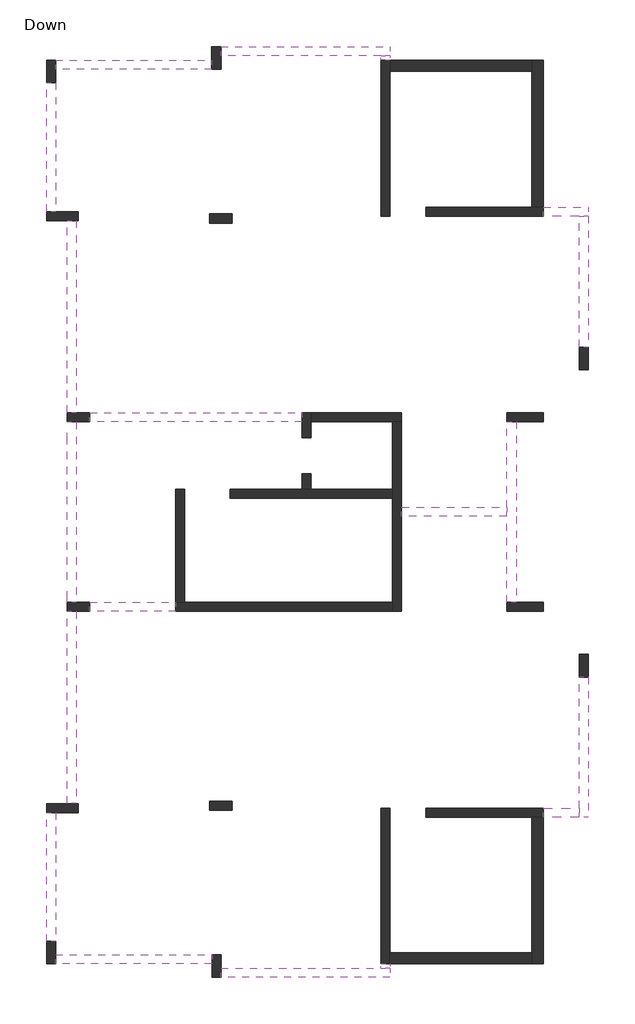
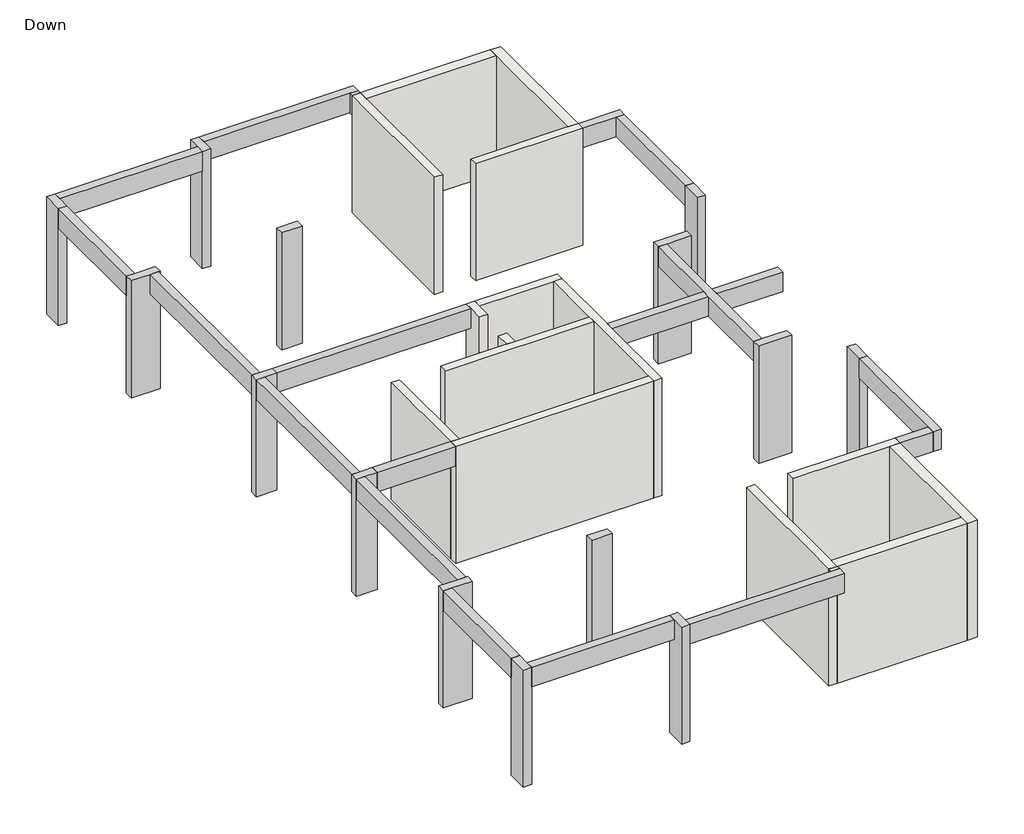
# One storey: 19 beams, 15 walls, 14 columns.
"""IFC4 building model written with IfcOpenShell, lengths in millimetres."""

from ifc_helpers import new_model, si_unit, origin, origin_with_axes, place, context, project, spatial, polyline, outline, extrude, faceted_brep, element, save

model = new_model("IFC4")

# Units and contexts
model_context = context("Model", 3, world=origin())
ifc_project = project(units=[si_unit("LENGTHUNIT", "METRE", prefix="MILLI")], contexts=[model_context])

# Site, building, storey
site = spatial("IfcSite", under=ifc_project)
building = spatial("IfcBuilding", under=site)
storey = spatial("IfcBuildingStorey", under=building, Name="Down", Elevation=0.0)

# Beams
placement = place(None, origin())
element("IfcBeam", 1, ObjectType="Concrete Rectengular Beam : 20/50", at=placement, inside=storey, context=model_context, shape_type="Brep", body=[
    faceted_brep([(-1347.6312201, 19838.1909584, 3000.0), (-1547.6312201, 19838.1909584, 3000.0), (-1547.6312201, 16987.4100295, 3000.0), (-1347.6312201, 16987.4100295, 3000.0), (-1547.6312201, 19838.1909584, 2500.0), (-1547.6312201, 16987.4100295, 2500.0), (-1347.6312201, 19838.1909584, 2500.0), (-1347.6312201, 16987.4100295, 2500.0), (-1347.6312201, 16987.4100295, 2800.0)], [[[0, 1, 2, 3]], [[1, 4, 5, 2]], [[4, 6, 7, 5]], [[6, 0, 3, 8, 7]], [[1, 0, 6, 4]], [[3, 2, 5, 7, 8]]]),
])
element("IfcBeam", 2, ObjectType="Concrete Rectengular Beam : 20/50", at=placement, inside=storey, context=model_context, shape_type="Brep", body=[
    faceted_brep([(-1086.1844466, 12537.0195651, 3000.0), (-886.1844466, 12537.0195651, 3000.0), (-886.1844466, 16787.4100295, 3000.0), (-1086.1844466, 16787.4100295, 3000.0), (-886.1844466, 12537.0195651, 2800.0), (-886.1844466, 12537.0195651, 2500.0), (-886.1844466, 16787.4100295, 2500.0), (-886.1844466, 16787.4100295, 2800.0), (-1086.1844466, 12537.0195651, 2500.0), (-1086.1844466, 16787.4100295, 2500.0), (-1086.1844466, 16787.4100295, 2800.0)], [[[0, 1, 2, 3]], [[2, 1, 4, 5, 6, 7]], [[5, 8, 9, 6]], [[3, 10, 9, 8, 0]], [[1, 0, 8, 5, 4]], [[3, 2, 7, 6, 9, 10]]]),
])
element("IfcBeam", 3, ObjectType="Concrete Rectengular Beam : 20/50", at=placement, inside=storey, context=model_context, shape_type="Brep", body=[
    faceted_brep([(-886.1844466, 12337.0195651, 3000.0), (-1086.1844466, 12337.0195651, 3000.0), (-1086.1844466, 11837.4100295, 3000.0), (-1086.1844466, 8836.9784636, 3000.0), (-1086.1844466, 8336.34139, 3000.0), (-886.1844466, 8336.34139, 3000.0), (-1086.1844466, 12337.0195651, 2500.0), (-1086.1844466, 8336.34139, 2500.0), (-886.1844466, 12337.0195651, 2500.0), (-886.1844466, 8336.34139, 2500.0), (-886.1844466, 12337.0195651, 2800.0), (-886.1844466, 8336.34139, 2800.0)], [[[0, 1, 2, 3, 4, 5]], [[1, 6, 7, 4, 3, 2]], [[6, 8, 9, 7]], [[8, 10, 0, 5, 11, 9]], [[1, 0, 10, 8, 6]], [[5, 4, 7, 9, 11]]]),
])
element("IfcBeam", 4, ObjectType="Concrete Rectengular Beam : 20/50", at=placement, inside=storey, context=model_context, shape_type="Brep", body=[
    faceted_brep([(-1086.1844466, 3886.9784636, 3000.0), (-886.1844466, 3886.9784636, 3000.0), (-886.1844466, 8136.34139, 3000.0), (-1086.1844466, 8136.34139, 3000.0), (-1086.1844466, 3886.9784636, 2500.0), (-1086.1844466, 3886.9784636, 2800.0), (-1086.1844466, 8136.34139, 2500.0), (-886.1844466, 3886.9784636, 2500.0), (-886.1844466, 8136.34139, 2500.0), (-886.1844466, 3886.9784636, 2800.0), (-886.1844466, 8136.34139, 2800.0)], [[[0, 1, 2, 3]], [[4, 5, 0, 3, 6]], [[7, 4, 6, 8]], [[2, 1, 9, 7, 8, 10]], [[3, 2, 10, 8, 6]], [[1, 0, 5, 4, 7, 9]]]),
])
element("IfcBeam", 5, ObjectType="Concrete Rectengular Beam : 20/50", at=placement, inside=storey, context=model_context, shape_type="Brep", body=[
    faceted_brep([(-1547.6312201, 836.1975347, 3000.0), (-1347.6312201, 836.1975347, 3000.0), (-1347.6312201, 3686.9784636, 3000.0), (-1547.6312201, 3686.9784636, 3000.0), (-1547.6312201, 3686.5951919, 3000.0), (-1347.6312201, 836.1975347, 2500.0), (-1347.6312201, 3686.9784636, 2500.0), (-1347.6312201, 3686.9784636, 2800.0), (-1547.6312201, 836.1975347, 2500.0), (-1547.6312201, 3686.9784636, 2500.0), (-1547.6312201, 3686.9784636, 2800.0)], [[[0, 1, 2, 3, 4]], [[1, 5, 6, 7, 2]], [[5, 8, 9, 6]], [[8, 0, 4, 3, 10, 9]], [[1, 0, 8, 5]], [[3, 2, 7, 6, 9, 10]]]),
])
element("IfcBeam", 6, ObjectType="Concrete Rectengular Beam : 20/50", at=placement, inside=storey, context=model_context, shape_type="Brep", body=[
    faceted_brep([(-1347.6312201, 537.7388417, 3000.0), (-1347.6312201, 337.7388417, 3000.0), (2114.3087716, 337.7388417, 3000.0), (2114.3087716, 537.7388417, 3000.0), (2114.3087716, 537.7388417, 2800.0), (2114.3087716, 537.7388417, 2500.0), (-1347.6312201, 537.7388417, 2500.0), (-1347.6312201, 537.7388417, 2800.0), (-1347.6312201, 337.7388417, 2500.0), (2114.3087716, 337.7388417, 2500.0)], [[[0, 1, 2, 3]], [[0, 3, 4, 5, 6, 7]], [[8, 6, 5, 9]], [[1, 8, 9, 2]], [[1, 0, 7, 6, 8]], [[3, 2, 9, 5, 4]]]),
])
element("IfcBeam", 7, ObjectType="Concrete Rectengular Beam : 20/50", at=placement, inside=storey, context=model_context, shape_type="Brep", body=[
    faceted_brep([(6055.3348071, 37.7388417, 3000.0), (6055.3348071, 237.7388417, 3000.0), (5855.3348071, 237.7388417, 3000.0), (2314.3087716, 237.7388417, 3000.0), (2314.3087716, 37.7388417, 3000.0), (6055.3348071, 37.7388417, 2500.0), (2314.3087716, 37.7388417, 2500.0), (6055.3348071, 237.7388417, 2500.0), (2314.3087716, 237.7388417, 2500.0), (5855.3348071, 237.7388417, 2500.0)], [[[0, 1, 2, 3, 4]], [[5, 0, 4, 6]], [[7, 5, 6, 8, 9]], [[1, 7, 9, 8, 3, 2]], [[4, 3, 8, 6]], [[1, 0, 5, 7]]]),
])
element("IfcBeam", 8, ObjectType="Concrete Rectengular Beam : 20/50", at=placement, inside=storey, context=model_context, shape_type="Brep", body=[
    faceted_brep([(2113.2812336, 20138.1909584, 3000.0), (2113.2812336, 20338.1909584, 3000.0), (-1347.6312201, 20338.1909584, 3000.0), (-1347.6312201, 20138.1909584, 3000.0), (2113.2812336, 20138.1909584, 2500.0), (2113.2812336, 20138.1909584, 2800.0), (-1347.6312201, 20138.1909584, 2800.0), (-1347.6312201, 20138.1909584, 2500.0), (2113.2812336, 20338.1909584, 2500.0), (-1347.6312201, 20338.1909584, 2500.0)], [[[0, 1, 2, 3]], [[4, 5, 0, 3, 6, 7]], [[8, 4, 7, 9]], [[1, 8, 9, 2]], [[1, 0, 5, 4, 8]], [[3, 2, 9, 7, 6]]]),
])
element("IfcBeam", 9, ObjectType="Concrete Rectengular Beam : 20/50", at=placement, inside=storey, context=model_context, shape_type="Brep", body=[
    faceted_brep([(6055.3348071, 20438.1909584, 3000.0), (6055.3348071, 20638.1909584, 3000.0), (2313.2812336, 20638.1909584, 3000.0), (2313.2812336, 20438.1909584, 3000.0), (5855.3348071, 20438.1909584, 3000.0), (6055.3348071, 20438.1909584, 2500.0), (2313.2812336, 20438.1909584, 2800.0), (2313.2812336, 20438.1909584, 2500.0), (5855.3348071, 20438.1909584, 2500.0), (6055.3348071, 20638.1909584, 2500.0), (2313.2812336, 20638.1909584, 2500.0)], [[[0, 1, 2, 3, 4]], [[5, 0, 4, 3, 6, 7, 8]], [[9, 5, 8, 7, 10]], [[1, 9, 10, 2]], [[3, 2, 10, 7, 6]], [[1, 0, 5, 9]]]),
])
element("IfcBeam", 10, ObjectType="Concrete Rectengular Beam : 20/50", at=placement, inside=storey, context=model_context, shape_type="Brep", body=[
    faceted_brep([(6055.3348071, 20438.1909584, 3000.0), (5855.3348071, 20438.1909584, 3000.0), (5855.3348071, 20337.1634204, 3000.0), (6055.3348071, 20337.1634204, 3000.0), (6055.3348071, 20438.1909584, 2500.0), (6055.3348071, 20337.1634204, 2500.0), (5855.3348071, 20438.1909584, 2500.0), (5855.3348071, 20337.1634204, 2500.0), (5855.3348071, 20438.1909584, 2800.0), (5855.3348071, 20337.1634204, 2800.0)], [[[0, 1, 2, 3]], [[4, 0, 3, 5]], [[6, 4, 5, 7]], [[2, 1, 8, 6, 7, 9]], [[1, 0, 4, 6, 8]], [[3, 2, 9, 7, 5]]]),
])
element("IfcBeam", 11, ObjectType="Concrete Rectengular Beam : 20/50", at=placement, inside=storey, context=model_context, shape_type="Brep", body=[
    faceted_brep([(5855.3348071, 237.7388417, 3000.0), (6055.3348071, 237.7388417, 3000.0), (6055.3348071, 336.1975347, 3000.0), (5855.3348071, 336.1975347, 3000.0), (5855.3348071, 336.1975347, 2800.0), (5855.3348071, 336.1975347, 2500.0), (5855.3348071, 237.7388417, 2500.0), (5855.3348071, 237.7388417, 2800.0), (6055.3348071, 237.7388417, 2500.0), (6055.3348071, 336.1975347, 2500.0)], [[[0, 1, 2, 3]], [[0, 3, 4, 5, 6, 7]], [[8, 6, 5, 9]], [[1, 8, 9, 2]], [[1, 0, 7, 6, 8]], [[3, 2, 9, 5, 4]]]),
])
element("IfcBeam", 12, ObjectType="Concrete Rectengular Beam : 20/50", at=placement, inside=storey, context=model_context, shape_type="Brep", body=[
    faceted_brep([(9453.0058534, 17086.8962605, 3000.0), (9453.0058534, 16886.8962605, 3000.0), (10255.2560168, 16886.8962605, 3000.0), (10455.2560168, 16886.8962605, 3000.0), (10455.2560168, 17086.8962605, 3000.0), (9453.0058534, 17086.8962605, 2500.0), (10455.2560168, 17086.8962605, 2500.0), (9453.0058534, 16886.8962605, 2500.0), (10455.2560168, 16886.8962605, 2500.0), (10255.2560168, 16886.8962605, 2500.0), (9453.0058534, 16886.8962605, 2800.0)], [[[0, 1, 2, 3, 4]], [[5, 0, 4, 6]], [[7, 5, 6, 8, 9]], [[8, 3, 2, 1, 10, 7, 9]], [[1, 0, 5, 7, 10]], [[4, 3, 8, 6]]]),
])
element("IfcBeam", 13, ObjectType="Concrete Rectengular Beam : 20/50", at=placement, inside=storey, context=model_context, shape_type="Brep", body=[
    faceted_brep([(-586.1844466, 8336.34139, 3000.0), (-586.1844466, 8136.34139, 3000.0), (1314.1854671, 8136.34139, 3000.0), (1314.1854671, 8336.34139, 3000.0), (-586.1844466, 8136.34139, 2800.0), (-586.1844466, 8136.34139, 2500.0), (1314.1854671, 8136.34139, 2500.0), (1314.1854671, 8136.34139, 2800.0), (-586.1844466, 8336.34139, 2500.0), (1314.1854671, 8336.34139, 2500.0), (1314.1854671, 8336.34139, 2800.0)], [[[0, 1, 2, 3]], [[2, 1, 4, 5, 6, 7]], [[5, 8, 9, 6]], [[8, 0, 3, 10, 9]], [[1, 0, 8, 5, 4]], [[3, 2, 7, 6, 9, 10]]]),
])
element("IfcBeam", 14, ObjectType="Concrete Rectengular Beam : 20/50", at=placement, inside=storey, context=model_context, shape_type="Brep", body=[
    faceted_brep([(-586.1844466, 12537.0195651, 3000.0), (-586.1844466, 12337.0195651, 3000.0), (4114.617033, 12337.0195651, 3000.0), (4114.617033, 12537.0195651, 3000.0), (-586.1844466, 12337.0195651, 2500.0), (4114.617033, 12337.0195651, 2500.0), (4114.617033, 12337.0195651, 2800.0), (-586.1844466, 12537.0195651, 2500.0), (4114.617033, 12537.0195651, 2500.0), (4114.617033, 12537.0195651, 2800.0), (-586.1844466, 12537.0195651, 2800.0)], [[[0, 1, 2, 3]], [[1, 4, 5, 6, 2]], [[4, 7, 8, 5]], [[0, 3, 9, 8, 7, 10]], [[1, 0, 10, 7, 4]], [[3, 2, 6, 5, 8, 9]]]),
])
element("IfcBeam", 15, ObjectType="Concrete Rectengular Beam : 20/50", at=placement, inside=storey, context=model_context, shape_type="Brep", body=[
    faceted_brep([(10255.2458863, 3586.4646946, 3000.0), (10455.2458863, 3586.4646946, 3000.0), (10455.2458863, 6686.3824915, 3000.0), (10255.2458863, 6686.3824915, 3000.0), (10255.2458863, 3786.4646946, 3000.0), (10255.2458863, 3586.4646946, 2500.0), (10255.2458863, 6686.3824915, 2500.0), (10255.2458863, 3786.4646946, 2500.0), (10455.2458863, 3586.4646946, 2500.0), (10455.2458863, 6686.3824915, 2500.0)], [[[0, 1, 2, 3, 4]], [[5, 0, 4, 3, 6, 7]], [[8, 5, 7, 6, 9]], [[1, 8, 9, 2]], [[3, 2, 9, 6]], [[1, 0, 5, 8]]]),
])
element("IfcBeam", 16, ObjectType="Concrete Rectengular Beam : 20/50", at=placement, inside=storey, context=model_context, shape_type="Brep", body=[
    faceted_brep([(10255.2458863, 3586.4646946, 3000.0), (10255.2458863, 3786.4646946, 3000.0), (9453.0058534, 3786.4646946, 3000.0), (9453.0058534, 3586.4646946, 3000.0), (10255.2458863, 3786.4646946, 2800.0), (10255.2458863, 3786.4646946, 2500.0), (9453.0058534, 3786.4646946, 2500.0), (9453.0058534, 3786.4646946, 2800.0), (10255.2458863, 3586.4646946, 2500.0), (9453.0058534, 3586.4646946, 2500.0)], [[[0, 1, 2, 3]], [[2, 1, 4, 5, 6, 7]], [[5, 8, 9, 6]], [[8, 0, 3, 9]], [[1, 0, 8, 5, 4]], [[3, 2, 7, 6, 9]]]),
])
element("IfcBeam", 17, ObjectType="Concrete Rectengular Beam : 20/50", at=placement, inside=storey, context=model_context, shape_type="Brep", body=[
    faceted_brep([(8852.8825489, 12337.0195651, 3000.0), (8652.8825489, 12337.0195651, 3000.0), (8652.8825489, 10438.2526107, 3000.0), (8652.8825489, 10238.2526107, 3000.0), (8652.8825489, 8336.34139, 3000.0), (8852.561957, 8336.34139, 3000.0), (8852.561957, 10238.2526107, 3000.0), (8852.8825489, 10238.2526107, 3000.0), (8852.8825489, 10438.2526107, 3000.0), (8852.8825489, 8336.34139, 2500.0), (8852.8825489, 10238.2526107, 2500.0), (8852.8825489, 10438.2526107, 2500.0), (8852.8825489, 12337.0195651, 2500.0), (8852.8825489, 12337.0195651, 2800.0), (8852.8825489, 10238.2526107, 2800.0), (8852.8825489, 8336.34139, 2800.0), (8652.8825489, 8336.34139, 2500.0), (8652.8825489, 10238.2526107, 2500.0), (8652.8825489, 10438.2526107, 2500.0), (8652.8825489, 12337.0195651, 2500.0), (8652.8825489, 8336.34139, 2800.0), (8652.8825489, 12337.0195651, 2800.0), (8852.561957, 8336.34139, 2800.0), (8852.561957, 10238.2526107, 2800.0)], [[[0, 1, 2, 3, 4, 5, 6, 7, 8]], [[9, 10, 11, 12, 13, 0, 8, 7, 14, 15]], [[9, 16, 17, 18, 19, 12, 11, 10]], [[19, 18, 17, 16, 20, 4, 3, 2, 1, 21]], [[16, 9, 15, 22, 5, 4, 20]], [[1, 0, 13, 12, 19, 21]], [[23, 22, 15, 14]], [[22, 23, 6, 5]], [[6, 23, 14, 7]]]),
])
element("IfcBeam", 18, ObjectType="Concrete Rectengular Beam : 20/50", at=placement, inside=storey, context=model_context, shape_type="Brep", body=[
    faceted_brep([(10453.8977564, 10238.2526107, 3000.0), (10453.8977564, 10238.2526107, 2800.0), (10453.8977564, 10238.2526107, 2500.0), (10453.8977564, 10438.2526107, 2500.0), (10453.8977564, 10438.2526107, 2800.0), (10453.8977564, 10438.2526107, 3000.0), (8852.8825489, 10238.2526107, 3000.0), (8852.8825489, 10438.2526107, 3000.0), (8852.8825489, 10438.2526107, 2800.0), (8852.8825489, 10438.2526107, 2500.0), (8852.8825489, 10238.2526107, 2500.0), (8852.8825489, 10238.2526107, 2800.0)], [[[0, 1, 2, 3, 4, 5]], [[6, 7, 8, 9, 10, 11]], [[0, 5, 7, 6]], [[5, 4, 3, 9, 8, 7]], [[3, 2, 10, 9]], [[2, 1, 0, 6, 11, 10]]]),
    faceted_brep([(6313.8977564, 10438.2526107, 3000.0), (6313.8977564, 10238.2526107, 3000.0), (8652.8825489, 10238.2526107, 3000.0), (8652.8825489, 10438.2526107, 3000.0), (6313.8977564, 10438.2526107, 2500.0), (6313.8977564, 10438.2526107, 2800.0), (8652.8825489, 10438.2526107, 2800.0), (8652.8825489, 10438.2526107, 2500.0), (6313.8977564, 10238.2526107, 2500.0), (8652.8825489, 10238.2526107, 2500.0)], [[[0, 1, 2, 3]], [[4, 5, 0, 3, 6, 7]], [[8, 4, 7, 9]], [[1, 8, 9, 2]], [[1, 0, 5, 4, 8]], [[3, 2, 9, 7, 6]]]),
])
element("IfcBeam", 19, ObjectType="Concrete Rectengular Beam : 20/50", at=placement, inside=storey, context=model_context, shape_type="Brep", body=[
    faceted_brep([(10255.2560168, 13985.039794, 3000.0), (10455.2560168, 13985.039794, 3000.0), (10455.2560168, 16886.8962605, 3000.0), (10255.2560168, 16886.8962605, 3000.0), (10455.2560168, 13985.039794, 2500.0), (10455.2560168, 16886.8962605, 2500.0), (10255.2560168, 13985.039794, 2500.0), (10255.2560168, 16886.8962605, 2500.0), (10255.2560168, 16886.8962605, 2800.0)], [[[0, 1, 2, 3]], [[1, 4, 5, 2]], [[4, 6, 7, 5]], [[6, 0, 3, 8, 7]], [[1, 0, 6, 4]], [[3, 2, 5, 7, 8]]]),
])

# Columns
element("IfcColumn", 20, ObjectType="Concrete Rectengular Column : 20/50", at=placement, inside=storey, context=model_context, shape_type="Brep", body=[
    faceted_brep([(-1347.6312201, 20338.1909584, 0.0), (-1347.6312201, 19838.1909584, 0.0), (-1547.6312201, 19838.1909584, 0.0), (-1547.6312201, 20338.1909584, 0.0), (-1347.6312201, 20338.1909584, 3000.0), (-1347.6312201, 20138.1909584, 3000.0), (-1347.6312201, 19838.1909584, 3000.0), (-1547.6312201, 19838.1909584, 3000.0), (-1547.6312201, 20338.1909584, 3000.0)], [[[0, 1, 2, 3]], [[4, 5, 6, 1, 0]], [[6, 7, 2, 1]], [[7, 8, 3, 2]], [[8, 4, 0, 3]], [[4, 8, 7, 6, 5]]]),
])
element("IfcColumn", 21, ObjectType="Concrete Rectengular Column : 20/50", at=placement, inside=storey, context=model_context, shape_type="Brep", body=[
    faceted_brep([(2313.2812336, 20638.1909584, 0.0), (2313.2812336, 20138.1909584, 0.0), (2113.2812336, 20138.1909584, 0.0), (2113.2812336, 20638.1909584, 0.0), (2313.2812336, 20638.1909584, 3000.0), (2313.2812336, 20438.1909584, 3000.0), (2313.2812336, 20138.1909584, 3000.0), (2313.2812336, 20138.1909584, 2800.0), (2113.2812336, 20138.1909584, 3000.0), (2113.2812336, 20638.1909584, 3000.0)], [[[0, 1, 2, 3]], [[4, 5, 6, 7, 1, 0]], [[6, 8, 2, 1, 7]], [[8, 9, 3, 2]], [[9, 4, 0, 3]], [[4, 9, 8, 6, 5]]]),
])
element("IfcColumn", 22, ObjectType="Concrete Rectengular Column : 20/50", at=placement, inside=storey, context=model_context, shape_type="Brep", body=[
    faceted_brep([(2063.507292, 16933.4642836, 0.0), (2563.507292, 16933.4642836, 0.0), (2563.507292, 16733.4642836, 0.0), (2063.507292, 16733.4642836, 0.0), (2063.507292, 16933.4642836, 3000.0), (2563.507292, 16933.4642836, 3000.0), (2563.507292, 16933.4642836, 2800.0), (2063.507292, 16933.4642836, 2800.0), (2563.507292, 16733.4642836, 3000.0), (2563.507292, 16733.4642836, 2800.0), (2063.507292, 16733.4642836, 3000.0), (2063.507292, 16733.4642836, 2800.0)], [[[0, 1, 2, 3]], [[4, 5, 6, 1, 0, 7]], [[5, 8, 9, 2, 1, 6]], [[8, 10, 11, 3, 2, 9]], [[10, 4, 7, 0, 3, 11]], [[4, 10, 8, 5]]]),
])
element("IfcColumn", 23, ObjectType="Concrete Rectengular Column : 20/50", at=placement, inside=storey, context=model_context, shape_type="Brep", body=[
    faceted_brep([(-1086.1844466, 12537.0195651, 0.0), (-586.1844466, 12537.0195651, 0.0), (-586.1844466, 12337.0195651, 0.0), (-1086.1844466, 12337.0195651, 0.0), (-1086.1844466, 12537.0195651, 3000.0), (-886.1844466, 12537.0195651, 3000.0), (-586.1844466, 12537.0195651, 3000.0), (-586.1844466, 12337.0195651, 3000.0), (-886.1844466, 12337.0195651, 3000.0), (-1086.1844466, 12337.0195651, 3000.0)], [[[0, 1, 2, 3]], [[4, 5, 6, 1, 0]], [[6, 7, 2, 1]], [[7, 8, 9, 3, 2]], [[9, 4, 0, 3]], [[4, 9, 8, 7, 6, 5]]]),
])
element("IfcColumn", 24, ObjectType="Concrete Rectengular Column : 20/50", at=placement, inside=storey, context=model_context, shape_type="Brep", body=[
    faceted_brep([(-1086.1844466, 8336.34139, 0.0), (-586.1844466, 8336.34139, 0.0), (-586.1844466, 8136.34139, 0.0), (-1086.1844466, 8136.34139, 0.0), (-1086.1844466, 8336.34139, 3000.0), (-886.1844466, 8336.34139, 3000.0), (-586.1844466, 8336.34139, 3000.0), (-586.1844466, 8136.34139, 3000.0), (-886.3077512, 8136.34139, 3000.0), (-1086.1844466, 8136.34139, 3000.0)], [[[0, 1, 2, 3]], [[4, 5, 6, 1, 0]], [[6, 7, 2, 1]], [[7, 8, 9, 3, 2]], [[9, 4, 0, 3]], [[4, 9, 8, 7, 6, 5]]]),
])
element("IfcColumn", 25, ObjectType="Concrete Rectengular Column : 20/50", at=placement, inside=storey, context=model_context, shape_type="Brep", body=[
    faceted_brep([(-1547.6312201, 336.1975347, 0.0), (-1547.6312201, 836.1975347, 0.0), (-1347.6312201, 836.1975347, 0.0), (-1347.6312201, 336.1975347, 0.0), (-1547.6312201, 336.1975347, 3000.0), (-1547.6312201, 836.1975347, 3000.0), (-1347.6312201, 836.1975347, 3000.0), (-1347.6312201, 537.7388417, 3000.0), (-1347.6312201, 336.1975347, 3000.0)], [[[0, 1, 2, 3]], [[4, 5, 1, 0]], [[5, 6, 2, 1]], [[6, 7, 8, 3, 2]], [[8, 4, 0, 3]], [[4, 8, 7, 6, 5]]]),
])
element("IfcColumn", 26, ObjectType="Concrete Rectengular Column : 20/50", at=placement, inside=storey, context=model_context, shape_type="Brep", body=[
    faceted_brep([(2566.6823845, 3734.6356769, 0.0), (2066.6823845, 3734.6356769, 0.0), (2066.6823845, 3934.6356769, 0.0), (2566.6823845, 3934.6356769, 0.0), (2566.6823845, 3734.6356769, 3000.0), (2066.6823845, 3734.6356769, 3000.0), (2066.6823845, 3734.6356769, 2800.0), (2566.6823845, 3734.6356769, 2800.0), (2066.6823845, 3934.6356769, 3000.0), (2066.6823845, 3934.6356769, 2800.0), (2566.6823845, 3934.6356769, 3000.0), (2566.6823845, 3934.6356769, 2800.0)], [[[0, 1, 2, 3]], [[4, 5, 6, 1, 0, 7]], [[5, 8, 9, 2, 1, 6]], [[8, 10, 11, 3, 2, 9]], [[10, 4, 7, 0, 3, 11]], [[4, 10, 8, 5]]]),
])
element("IfcColumn", 27, ObjectType="Concrete Rectengular Column : 20/50", at=placement, inside=storey, context=model_context, shape_type="Brep", body=[
    faceted_brep([(2314.3087716, 537.7388417, 0.0), (2314.3087716, 37.7388417, 0.0), (2114.3087716, 37.7388417, 0.0), (2114.3087716, 537.7388417, 0.0), (2314.3087716, 537.7388417, 3000.0), (2314.3087716, 237.7388417, 3000.0), (2314.3087716, 37.7388417, 3000.0), (2314.3087716, 537.7388417, 2800.0), (2114.3087716, 37.7388417, 3000.0), (2114.3087716, 537.7388417, 3000.0)], [[[0, 1, 2, 3]], [[4, 5, 6, 1, 0, 7]], [[6, 8, 2, 1]], [[8, 9, 3, 2]], [[9, 4, 7, 0, 3]], [[4, 9, 8, 6, 5]]]),
])
element("IfcColumn", 28, ObjectType="Concrete Rectengular Column : 20/50", at=placement, inside=storey, context=model_context, shape_type="SweptSolid", body=[
    extrude(outline(polyline([(10455.2458863, 7186.3824915), (10455.2458863, 6686.3824915), (10255.2458863, 6686.3824915), (10255.2458863, 7186.3824915), (10455.2458863, 7186.3824915)])), origin_with_axes(), (0.0, 0.0, 1.0), 3000.0),
])
element("IfcColumn", 29, ObjectType="Concrete Rectengular Column : 20/50", at=placement, inside=storey, context=model_context, shape_type="Brep", body=[
    faceted_brep([(10455.2560168, 13985.039794, 0.0), (10455.2560168, 13485.039794, 0.0), (10255.2560168, 13485.039794, 0.0), (10255.2560168, 13985.039794, 0.0), (10455.2560168, 13985.039794, 3000.0), (10455.2560168, 13485.039794, 3000.0), (10255.2560168, 13485.039794, 3000.0), (10255.2560168, 13485.039794, 2800.0), (10255.2560168, 13985.039794, 3000.0)], [[[0, 1, 2, 3]], [[4, 5, 1, 0]], [[5, 6, 7, 2, 1]], [[6, 8, 3, 2, 7]], [[8, 4, 0, 3]], [[4, 8, 6, 5]]]),
])
element("IfcColumn", 30, ObjectType="Concrete Rectengular Column : 20/70", at=placement, inside=storey, context=model_context, shape_type="Brep", body=[
    faceted_brep([(-1547.6312201, 16987.4100295, 0.0), (-847.6312201, 16987.4100295, 0.0), (-847.6312201, 16787.4100295, 0.0), (-1547.6312201, 16787.4100295, 0.0), (-1547.6312201, 16987.4100295, 3000.0), (-1347.6312201, 16987.4100295, 3000.0), (-847.6312201, 16987.4100295, 3000.0), (-847.6312201, 16987.4100295, 2800.0), (-1547.6312201, 16987.4100295, 2800.0), (-847.6312201, 16787.4100295, 3000.0), (-847.6312201, 16787.4100295, 2800.0), (-886.1844466, 16787.4100295, 3000.0), (-1086.1844466, 16787.4100295, 3000.0), (-1547.6312201, 16787.4100295, 3000.0), (-1547.6312201, 16787.4100295, 2800.0)], [[[0, 1, 2, 3]], [[4, 5, 6, 7, 1, 0, 8]], [[6, 9, 10, 2, 1, 7]], [[9, 11, 12, 13, 14, 3, 2, 10]], [[13, 4, 8, 0, 3, 14]], [[4, 13, 12, 11, 9, 6, 5]]]),
])
element("IfcColumn", 31, ObjectType="Concrete Rectengular Column : 20/70", at=placement, inside=storey, context=model_context, shape_type="Brep", body=[
    faceted_brep([(-1547.6312201, 3886.9784636, 0.0), (-847.6312201, 3886.9784636, 0.0), (-847.6312201, 3686.9784636, 0.0), (-1547.6312201, 3686.9784636, 0.0), (-1547.6312201, 3886.9784636, 3000.0), (-1086.1844466, 3886.9784636, 3000.0), (-886.3077512, 3886.9784636, 3000.0), (-847.6312201, 3886.9784636, 3000.0), (-847.6312201, 3886.9784636, 2800.0), (-1547.6312201, 3886.9784636, 2800.0), (-847.6312201, 3686.9784636, 3000.0), (-847.6312201, 3686.9784636, 2800.0), (-1347.7545247, 3686.9784636, 3000.0), (-1547.6312201, 3686.9784636, 3000.0)], [[[0, 1, 2, 3]], [[4, 5, 6, 7, 8, 1, 0, 9]], [[7, 10, 11, 2, 1, 8]], [[10, 12, 13, 3, 2, 11]], [[13, 4, 9, 0, 3]], [[4, 13, 12, 10, 7, 6, 5]]]),
])
element("IfcColumn", 32, ObjectType="Concrete Rectengular Column : 20/80", at=placement, inside=storey, context=model_context, shape_type="Brep", body=[
    faceted_brep([(8652.8825489, 8336.34139, 0.0), (9452.8825489, 8336.34139, 0.0), (9452.8825489, 8136.34139, 0.0), (8652.8825489, 8136.34139, 0.0), (8652.8825489, 8336.34139, 3000.0), (8852.561957, 8336.34139, 3000.0), (9452.8825489, 8336.34139, 3000.0), (9452.8825489, 8336.34139, 2800.0), (9452.8825489, 8136.34139, 3000.0), (9452.8825489, 8136.34139, 2800.0), (8652.8825489, 8136.34139, 3000.0), (8652.8825489, 8136.34139, 2800.0)], [[[0, 1, 2, 3]], [[4, 5, 6, 7, 1, 0]], [[6, 8, 9, 2, 1, 7]], [[8, 10, 11, 3, 2, 9]], [[10, 4, 0, 3, 11]], [[4, 10, 8, 6, 5]]]),
])
element("IfcColumn", 33, ObjectType="Concrete Rectengular Column : 20/80", at=placement, inside=storey, context=model_context, shape_type="Brep", body=[
    faceted_brep([(8652.8825489, 12537.0195651, 0.0), (9452.8825489, 12537.0195651, 0.0), (9452.8825489, 12337.0195651, 0.0), (8652.8825489, 12337.0195651, 0.0), (8652.8825489, 12537.0195651, 3000.0), (9452.8825489, 12537.0195651, 3000.0), (9452.8825489, 12537.0195651, 2800.0), (8652.8825489, 12537.0195651, 2800.0), (9452.8825489, 12337.0195651, 3000.0), (8852.8825489, 12337.0195651, 3000.0), (8652.8825489, 12337.0195651, 3000.0)], [[[0, 1, 2, 3]], [[4, 5, 6, 1, 0, 7]], [[5, 8, 2, 1, 6]], [[8, 9, 10, 3, 2]], [[10, 4, 7, 0, 3]], [[4, 10, 9, 8, 5]]]),
])

# Walls
element("IfcWall", 34, ObjectType="20", at=placement, inside=storey, context=model_context, shape_type="Brep", body=[
    faceted_brep([(6055.3348071, 16886.8962605, 0.0), (6055.3348071, 20087.1634204, 0.0), (6055.3348071, 20337.1634204, 0.0), (6055.3348071, 20337.1634204, 2500.0), (6055.3348071, 20337.1634204, 3000.0), (6055.3348071, 20087.1634204, 3000.0), (6055.3348071, 16986.8962605, 3000.0), (6055.3348071, 16886.8962605, 3000.0), (6055.3348071, 16886.8962605, 2800.0), (5855.3348071, 16886.8962605, 0.0), (5855.3348071, 16886.8962605, 2800.0), (5855.3348071, 16886.8962605, 3000.0), (5855.3348071, 20337.1634204, 3000.0), (5855.3348071, 20337.1634204, 2500.0), (5855.3348071, 20337.1634204, 0.0)], [[[0, 1, 2, 3, 4, 5, 6, 7, 8]], [[9, 10, 11, 12, 13, 14]], [[2, 1, 0, 9, 14]], [[7, 6, 5, 4, 12, 11]], [[0, 8, 7, 11, 10, 9]], [[4, 3, 2, 14, 13, 12]]]),
])
element("IfcWall", 35, ObjectType="20", at=placement, inside=storey, context=model_context, shape_type="Brep", body=[
    faceted_brep([(6853.6634778, 16886.8962605, 0.0), (9453.0058534, 16886.8962605, 0.0), (9453.0058534, 16886.8962605, 2500.0), (9453.0058534, 16886.8962605, 3000.0), (6853.6634778, 16886.8962605, 3000.0), (6853.6634778, 16886.8962605, 2800.0), (6853.6634778, 17086.8962605, 0.0), (6853.6634778, 17086.8962605, 2800.0), (6853.6634778, 17086.8962605, 3000.0), (9203.0058534, 17086.8962605, 3000.0), (9453.0058534, 17086.8962605, 3000.0), (9453.0058534, 17086.8962605, 2500.0), (9453.0058534, 17086.8962605, 0.0), (9203.0058534, 17086.8962605, 0.0), (6853.6634778, 16986.8962605, 3000.0)], [[[0, 1, 2, 3, 4, 5]], [[6, 7, 8, 9, 10, 11, 12, 13]], [[1, 0, 6, 13, 12]], [[4, 3, 10, 9, 8, 14]], [[0, 5, 4, 14, 8, 7, 6]], [[3, 2, 1, 12, 11, 10]]]),
])
element("IfcWall", 36, ObjectType="20", at=placement, inside=storey, context=model_context, shape_type="Brep", body=[
    faceted_brep([(5855.3348071, 3786.4646946, 0.0), (5855.3348071, 336.1975347, 0.0), (5855.3348071, 336.1975347, 2500.0), (5855.3348071, 336.1975347, 3000.0), (5855.3348071, 3786.4646946, 3000.0), (5855.3348071, 3786.4646946, 2800.0), (6055.3348071, 3786.4646946, 0.0), (6055.3348071, 3786.4646946, 2800.0), (6055.3348071, 3786.4646946, 3000.0), (6055.3348071, 3691.2119202, 3000.0), (6055.3348071, 586.1975347, 3000.0), (6055.3348071, 336.1975347, 3000.0), (6055.3348071, 336.1975347, 2500.0), (6055.3348071, 336.1975347, 0.0), (6055.3348071, 586.1975347, 0.0)], [[[0, 1, 2, 3, 4, 5]], [[6, 7, 8, 9, 10, 11, 12, 13, 14]], [[1, 0, 6, 14, 13]], [[4, 3, 11, 10, 9, 8]], [[0, 5, 4, 8, 7, 6]], [[3, 2, 1, 13, 12, 11]]]),
])
element("IfcWall", 37, ObjectType="20", at=placement, inside=storey, context=model_context, shape_type="Brep", body=[
    faceted_brep([(6853.6634778, 3586.4646946, 0.0), (9203.0058534, 3586.4646946, 0.0), (9453.0058534, 3586.4646946, 0.0), (9453.0058534, 3586.4646946, 2500.0), (9453.0058534, 3586.4646946, 3000.0), (9203.0058534, 3586.4646946, 3000.0), (6853.6634778, 3586.4646946, 3000.0), (6853.6634778, 3586.4646946, 2800.0), (6853.6634778, 3786.4646946, 0.0), (6853.6634778, 3786.4646946, 2800.0), (6853.6634778, 3786.4646946, 3000.0), (9453.0058534, 3786.4646946, 3000.0), (9453.0058534, 3786.4646946, 2500.0), (9453.0058534, 3786.4646946, 0.0), (6853.6634778, 3691.2119202, 3000.0)], [[[0, 1, 2, 3, 4, 5, 6, 7]], [[8, 9, 10, 11, 12, 13]], [[2, 1, 0, 8, 13]], [[6, 5, 4, 11, 10, 14]], [[0, 7, 6, 14, 10, 9, 8]], [[4, 3, 2, 13, 12, 11]]]),
])
element("IfcWall", 38, ObjectType="20", at=placement, inside=storey, context=model_context, shape_type="Brep", body=[
    faceted_brep([(4314.617033, 11986.6702022, 0.0), (4314.617033, 12337.0195651, 0.0), (4314.617033, 12537.0195651, 0.0), (4314.617033, 12537.0195651, 3000.0), (4314.617033, 12337.0195651, 3000.0), (4314.617033, 11986.6702022, 3000.0), (4114.617033, 11986.6702022, 0.0), (4114.617033, 11986.6702022, 2800.0), (4114.617033, 11986.6702022, 3000.0), (4114.617033, 12337.0195651, 3000.0), (4114.617033, 12537.0195651, 3000.0), (4114.617033, 12537.0195651, 0.0), (4214.617033, 11986.6702022, 3000.0)], [[[0, 1, 2, 3, 4, 5]], [[6, 7, 8, 9, 10, 11]], [[2, 1, 0, 6, 11]], [[5, 4, 3, 10, 9, 8, 12]], [[0, 5, 12, 8, 7, 6]], [[3, 2, 11, 10]]]),
])
element("IfcWall", 39, ObjectType="20", at=placement, inside=storey, context=model_context, shape_type="Brep", body=[
    faceted_brep([(4314.617033, 12337.0195651, 0.0), (6113.8977564, 12337.0195651, 0.0), (6313.8977564, 12337.0195651, 0.0), (6313.8977564, 12337.0195651, 3000.0), (6113.8977564, 12337.0195651, 3000.0), (4314.617033, 12337.0195651, 3000.0), (4314.617033, 12537.0195651, 0.0), (4314.617033, 12537.0195651, 3000.0), (6313.8977564, 12537.0195651, 3000.0), (6313.8977564, 12537.0195651, 2800.0), (6313.8977564, 12537.0195651, 0.0)], [[[0, 1, 2, 3, 4, 5]], [[6, 7, 8, 9, 10]], [[2, 1, 0, 6, 10]], [[5, 4, 3, 8, 7]], [[0, 5, 7, 6]], [[3, 2, 10, 9, 8]]]),
])
element("IfcWall", 40, ObjectType="20", at=placement, inside=storey, context=model_context, shape_type="Brep", body=[
    faceted_brep([(2514.3704239, 10637.286725, 0.0), (6113.8977564, 10637.286725, 0.0), (6113.8977564, 10637.286725, 3000.0), (2619.3704239, 10637.286725, 3000.0), (2514.3704239, 10637.286725, 3000.0), (2514.3704239, 10637.286725, 2800.0), (2514.3704239, 10837.286725, 0.0), (2514.3704239, 10837.286725, 2800.0), (2514.3704239, 10837.286725, 3000.0), (4114.617033, 10837.286725, 3000.0), (4314.617033, 10837.286725, 3000.0), (6113.8977564, 10837.286725, 3000.0), (6113.8977564, 10837.286725, 0.0), (4314.617033, 10837.286725, 0.0), (4114.617033, 10837.286725, 0.0), (2514.3704239, 10737.286725, 3000.0)], [[[0, 1, 2, 3, 4, 5]], [[6, 7, 8, 9, 10, 11, 12, 13, 14]], [[1, 0, 6, 14, 13, 12]], [[4, 3, 2, 11, 10, 9, 8, 15]], [[0, 5, 4, 15, 8, 7, 6]], [[2, 1, 12, 11]]]),
])
element("IfcWall", 41, ObjectType="20", at=placement, inside=storey, context=model_context, shape_type="Brep", body=[
    faceted_brep([(4114.617033, 11186.5468976, 0.0), (4114.617033, 10837.286725, 0.0), (4114.617033, 10837.286725, 2800.0), (4114.617033, 10837.286725, 3000.0), (4114.617033, 11186.5468976, 3000.0), (4114.617033, 11186.5468976, 2800.0), (4314.617033, 11186.5468976, 0.0), (4314.617033, 11186.5468976, 3000.0), (4314.617033, 10837.286725, 3000.0), (4314.617033, 10837.286725, 0.0), (4214.617033, 11186.5468976, 3000.0)], [[[0, 1, 2, 3, 4, 5]], [[6, 7, 8, 9]], [[1, 0, 6, 9]], [[4, 3, 8, 7, 10]], [[0, 5, 4, 10, 7, 6]], [[3, 2, 1, 9, 8]]]),
])
element("IfcWall", 42, ObjectType="20", at=placement, inside=storey, context=model_context, shape_type="Brep", body=[
    faceted_brep([(6113.8977564, 12337.0195651, 0.0), (6113.8977564, 10837.286725, 0.0), (6113.8977564, 10637.286725, 0.0), (6113.8977564, 8336.34139, 0.0), (6113.8977564, 8136.34139, 0.0), (6113.8977564, 8136.34139, 3000.0), (6113.8977564, 8336.34139, 3000.0), (6113.8977564, 10637.286725, 3000.0), (6113.8977564, 10837.286725, 3000.0), (6113.8977564, 12337.0195651, 3000.0), (6313.8977564, 12337.0195651, 0.0), (6313.8977564, 12337.0195651, 3000.0), (6313.8977564, 10438.2526107, 3000.0), (6313.8977564, 10238.2526107, 3000.0), (6313.8977564, 8136.34139, 3000.0), (6313.8977564, 8136.34139, 2800.0), (6313.8977564, 8136.34139, 0.0)], [[[0, 1, 2, 3, 4, 5, 6, 7, 8, 9]], [[10, 11, 12, 13, 14, 15, 16]], [[4, 3, 2, 1, 0, 10, 16]], [[9, 8, 7, 6, 5, 14, 13, 12, 11]], [[0, 9, 11, 10]], [[5, 4, 16, 15, 14]]]),
])
element("IfcWall", 43, ObjectType="20", at=placement, inside=storey, context=model_context, shape_type="Brep", body=[
    faceted_brep([(6113.8977564, 8336.34139, 0.0), (1514.1854671, 8336.34139, 0.0), (1314.1854671, 8336.34139, 0.0), (1314.1854671, 8336.34139, 2500.0), (1314.1854671, 8336.34139, 3000.0), (1514.1854671, 8336.34139, 3000.0), (2619.3704239, 8336.34139, 3000.0), (6113.8977564, 8336.34139, 3000.0), (6113.8977564, 8136.34139, 0.0), (6113.8977564, 8136.34139, 3000.0), (1314.1854671, 8136.34139, 3000.0), (1314.1854671, 8136.34139, 2500.0), (1314.1854671, 8136.34139, 0.0)], [[[0, 1, 2, 3, 4, 5, 6, 7]], [[8, 9, 10, 11, 12]], [[2, 1, 0, 8, 12]], [[7, 6, 5, 4, 10, 9]], [[0, 7, 9, 8]], [[4, 3, 2, 12, 11, 10]]]),
])
element("IfcWall", 44, ObjectType="20", at=placement, inside=storey, context=model_context, shape_type="Brep", body=[
    faceted_brep([(1514.1854671, 8336.34139, 0.0), (1514.1854671, 10837.286725, 0.0), (1514.1854671, 10837.286725, 2800.0), (1514.1854671, 10837.286725, 3000.0), (1514.1854671, 10737.286725, 3000.0), (1514.1854671, 8336.34139, 3000.0), (1514.1854671, 8336.34139, 2800.0), (1314.1854671, 8336.34139, 0.0), (1314.1854671, 8336.34139, 2800.0), (1314.1854671, 8336.34139, 3000.0), (1314.1854671, 10837.286725, 3000.0), (1314.1854671, 10837.286725, 2800.0), (1314.1854671, 10837.286725, 0.0)], [[[0, 1, 2, 3, 4, 5, 6]], [[7, 8, 9, 10, 11, 12]], [[1, 0, 7, 12]], [[3, 2, 1, 12, 11, 10]], [[5, 4, 3, 10, 9]], [[0, 6, 5, 9, 8, 7]]]),
])
element("IfcWall", 45, ObjectType="25", at=placement, inside=storey, context=model_context, shape_type="Brep", body=[
    faceted_brep([(9453.0058534, 17086.8962605, 0.0), (9453.0058534, 20337.1634204, 0.0), (9453.0058534, 20337.1634204, 3000.0), (9453.0058534, 17086.8962605, 3000.0), (9203.0058534, 17086.8962605, 0.0), (9203.0058534, 17086.8962605, 2800.0), (9203.0058534, 17086.8962605, 3000.0), (9203.0058534, 20087.1634204, 3000.0), (9203.0058534, 20337.1634204, 3000.0), (9203.0058534, 20337.1634204, 0.0), (9203.0058534, 20087.1634204, 0.0)], [[[0, 1, 2, 3]], [[4, 5, 6, 7, 8, 9, 10]], [[1, 0, 4, 10, 9]], [[3, 2, 8, 7, 6]], [[0, 3, 6, 5, 4]], [[2, 1, 9, 8]]]),
])
element("IfcWall", 46, ObjectType="25", at=placement, inside=storey, context=model_context, shape_type="Brep", body=[
    faceted_brep([(9203.0058534, 20337.1634204, 0.0), (6055.3348071, 20337.1634204, 0.0), (6055.3348071, 20337.1634204, 3000.0), (9203.0058534, 20337.1634204, 3000.0), (9203.0058534, 20087.1634204, 0.0), (9203.0058534, 20087.1634204, 2800.0), (9203.0058534, 20087.1634204, 3000.0), (6055.3348071, 20087.1634204, 3000.0), (6055.3348071, 20087.1634204, 2800.0), (6055.3348071, 20087.1634204, 0.0)], [[[0, 1, 2, 3]], [[4, 5, 6, 7, 8, 9]], [[1, 0, 4, 9]], [[3, 2, 7, 6]], [[0, 3, 6, 5, 4]], [[2, 1, 9, 8, 7]]]),
])
element("IfcWall", 47, ObjectType="25", at=placement, inside=storey, context=model_context, shape_type="Brep", body=[
    faceted_brep([(9203.0058534, 3586.4646946, 0.0), (9203.0058534, 586.1975347, 0.0), (9203.0058534, 336.1975347, 0.0), (9203.0058534, 336.1975347, 3000.0), (9203.0058534, 586.1975347, 3000.0), (9203.0058534, 3586.4646946, 3000.0), (9203.0058534, 3586.4646946, 2800.0), (9453.0058534, 3586.4646946, 0.0), (9453.0058534, 3586.4646946, 3000.0), (9453.0058534, 336.1975347, 3000.0), (9453.0058534, 336.1975347, 0.0)], [[[0, 1, 2, 3, 4, 5, 6]], [[7, 8, 9, 10]], [[2, 1, 0, 7, 10]], [[5, 4, 3, 9, 8]], [[0, 6, 5, 8, 7]], [[3, 2, 10, 9]]]),
])
element("IfcWall", 48, ObjectType="25", at=placement, inside=storey, context=model_context, shape_type="Brep", body=[
    faceted_brep([(9203.0058534, 586.1975347, 0.0), (6055.3348071, 586.1975347, 0.0), (6055.3348071, 586.1975347, 2800.0), (6055.3348071, 586.1975347, 3000.0), (9203.0058534, 586.1975347, 3000.0), (9203.0058534, 586.1975347, 2800.0), (9203.0058534, 336.1975347, 0.0), (9203.0058534, 336.1975347, 3000.0), (6055.3348071, 336.1975347, 3000.0), (6055.3348071, 336.1975347, 0.0)], [[[0, 1, 2, 3, 4, 5]], [[6, 7, 8, 9]], [[1, 0, 6, 9]], [[4, 3, 8, 7]], [[0, 5, 4, 7, 6]], [[3, 2, 1, 9, 8]]]),
])

save(model, "model.ifc")

# Revit data of these elements
# Project information
#   Project Issue Date = "Issue Date"
#   Project Status = "Project Status"
#   Client Name = "לקוח"
#   Project Address = "Enter address here"
#   Project Name = "Project 008"
#   Project Number = "מספר פרויקט"
# Type "Concrete Rectengular Beam : 20/50"
#   Length [instance default] = 152.4 cm
#   b = 20 cm
#   h = 50 cm
#   Structural Material [instance default] = Concrete
#   Assembly Code = ""
# Type "Concrete Rectengular Column : 20/50"
#   b = 20 cm
#   h = 50 cm
#   Structural Material [instance default] = Concrete
# Type "Concrete Rectengular Column : 20/70"
#   b = 20 cm
#   h = 70 cm
#   Structural Material [instance default] = Concrete
# Type "Concrete Rectengular Column : 20/80"
#   b = 20 cm
#   h = 80 cm
#   Structural Material [instance default] = Concrete
# Type "20"
#   Layers, outside or top first: 20 cm "Concrete" (function 1)
# Type "25"
#   Layers, outside or top first: 25 cm "Concrete" (function 1)
# Element 1 (IfcBeam, "Concrete Rectengular Beam : 20/50")
#   Comments = ""
#   Mark = "B1"
#   SOFiSTiK_AMG_Comments = ""
#   SOFiSTiK_AMG_Scheduled = yes
#   SOFiSTiK_AMG_Adjusted = yes
#   Structural Material = Concrete
#   Phase Created = New Construction
#   Materials on its faces: "Concrete"
# Element 2 (IfcBeam, "Concrete Rectengular Beam : 20/50")
#   Comments = ""
#   Mark = "B2"
#   SOFiSTiK_AMG_Comments = ""
#   SOFiSTiK_AMG_Scheduled = yes
#   SOFiSTiK_AMG_Adjusted = yes
#   Structural Material = Concrete
#   Phase Created = New Construction
#   Materials on its faces: "Concrete"
# Element 3 (IfcBeam, "Concrete Rectengular Beam : 20/50")
#   Comments = ""
#   Mark = "B3"
#   SOFiSTiK_AMG_Comments = ""
#   SOFiSTiK_AMG_Scheduled = yes
#   SOFiSTiK_AMG_Adjusted = yes
#   Structural Material = Concrete
#   Phase Created = New Construction
#   Materials on its faces: "Concrete"
# Element 4 (IfcBeam, "Concrete Rectengular Beam : 20/50")
#   Comments = ""
#   Mark = "B4"
#   SOFiSTiK_AMG_Comments = ""
#   SOFiSTiK_AMG_Scheduled = yes
#   SOFiSTiK_AMG_Adjusted = yes
#   Structural Material = Concrete
#   Phase Created = New Construction
#   Materials on its faces: "Concrete"
# Element 5 (IfcBeam, "Concrete Rectengular Beam : 20/50")
#   Comments = ""
#   Mark = "B5"
#   SOFiSTiK_AMG_Comments = ""
#   SOFiSTiK_AMG_Scheduled = yes
#   SOFiSTiK_AMG_Adjusted = yes
#   Structural Material = Concrete
#   Phase Created = New Construction
#   Materials on its faces: "Concrete"
# Element 6 (IfcBeam, "Concrete Rectengular Beam : 20/50")
#   Comments = ""
#   Mark = "B6"
#   SOFiSTiK_AMG_Comments = ""
#   SOFiSTiK_AMG_Scheduled = yes
#   SOFiSTiK_AMG_Adjusted = yes
#   Structural Material = Concrete
#   Phase Created = New Construction
#   Materials on its faces: "Concrete"
# Element 7 (IfcBeam, "Concrete Rectengular Beam : 20/50")
#   Comments = ""
#   Mark = "B7"
#   SOFiSTiK_AMG_Comments = ""
#   SOFiSTiK_AMG_Scheduled = yes
#   SOFiSTiK_AMG_Adjusted = yes
#   Structural Material = Concrete
#   Phase Created = New Construction
#   Materials on its faces: "Concrete"
# Element 8 (IfcBeam, "Concrete Rectengular Beam : 20/50")
#   Comments = ""
#   Mark = "B8"
#   SOFiSTiK_AMG_Comments = ""
#   SOFiSTiK_AMG_Scheduled = yes
#   SOFiSTiK_AMG_Adjusted = yes
#   Structural Material = Concrete
#   Phase Created = New Construction
#   Materials on its faces: "Concrete"
# Element 9 (IfcBeam, "Concrete Rectengular Beam : 20/50")
#   Comments = ""
#   Mark = "B9"
#   SOFiSTiK_AMG_Comments = ""
#   SOFiSTiK_AMG_Scheduled = yes
#   SOFiSTiK_AMG_Adjusted = yes
#   Structural Material = Concrete
#   Phase Created = New Construction
#   Materials on its faces: "Concrete"
# Element 10 (IfcBeam, "Concrete Rectengular Beam : 20/50")
#   Comments = ""
#   Mark = "B10"
#   SOFiSTiK_AMG_Comments = "Too Short Element /"
#   SOFiSTiK_AMG_Scheduled = yes
#   SOFiSTiK_AMG_Adjusted = yes
#   Structural Material = Concrete
#   Phase Created = New Construction
#   Materials on its faces: "Concrete"
# Element 11 (IfcBeam, "Concrete Rectengular Beam : 20/50")
#   Comments = ""
#   Mark = "B11"
#   SOFiSTiK_AMG_Comments = "Too Short Element /"
#   SOFiSTiK_AMG_Scheduled = yes
#   SOFiSTiK_AMG_Adjusted = yes
#   Structural Material = Concrete
#   Phase Created = New Construction
#   Materials on its faces: "Concrete"
# Element 12 (IfcBeam, "Concrete Rectengular Beam : 20/50")
#   Comments = ""
#   Mark = "B12"
#   SOFiSTiK_AMG_Comments = ""
#   SOFiSTiK_AMG_Scheduled = yes
#   SOFiSTiK_AMG_Adjusted = yes
#   Structural Material = Concrete
#   Phase Created = New Construction
#   Materials on its faces: "Concrete"
# Element 13 (IfcBeam, "Concrete Rectengular Beam : 20/50")
#   Comments = ""
#   Mark = "B13"
#   SOFiSTiK_AMG_Comments = ""
#   SOFiSTiK_AMG_Scheduled = yes
#   SOFiSTiK_AMG_Adjusted = yes
#   Structural Material = Concrete
#   Phase Created = New Construction
#   Materials on its faces: "Concrete"
# Element 14 (IfcBeam, "Concrete Rectengular Beam : 20/50")
#   Comments = ""
#   Mark = "B15"
#   SOFiSTiK_AMG_Comments = ""
#   SOFiSTiK_AMG_Scheduled = yes
#   SOFiSTiK_AMG_Adjusted = yes
#   Structural Material = Concrete
#   Phase Created = New Construction
#   Materials on its faces: "Concrete"
# Element 15 (IfcBeam, "Concrete Rectengular Beam : 20/50")
#   Comments = ""
#   Mark = "B16"
#   SOFiSTiK_AMG_Comments = ""
#   SOFiSTiK_AMG_Scheduled = yes
#   SOFiSTiK_AMG_Adjusted = yes
#   Structural Material = Concrete
#   Phase Created = New Construction
#   Materials on its faces: "Concrete"
# Element 16 (IfcBeam, "Concrete Rectengular Beam : 20/50")
#   Comments = ""
#   Mark = "B17"
#   SOFiSTiK_AMG_Comments = ""
#   SOFiSTiK_AMG_Scheduled = yes
#   SOFiSTiK_AMG_Adjusted = yes
#   Structural Material = Concrete
#   Phase Created = New Construction
#   Materials on its faces: "Concrete"
# Element 17 (IfcBeam, "Concrete Rectengular Beam : 20/50")
#   Comments = ""
#   Mark = "B18"
#   SOFiSTiK_AMG_Comments = ""
#   SOFiSTiK_AMG_Scheduled = yes
#   SOFiSTiK_AMG_Adjusted = yes
#   Structural Material = Concrete
#   Phase Created = New Construction
#   Materials on its faces: "Concrete"
# Element 18 (IfcBeam, "Concrete Rectengular Beam : 20/50")
#   Comments = ""
#   Mark = "B19"
#   SOFiSTiK_AMG_Comments = ""
#   SOFiSTiK_AMG_Scheduled = yes
#   SOFiSTiK_AMG_Adjusted = yes
#   Structural Material = Concrete
#   Phase Created = New Construction
#   Materials on its faces: "Concrete"
# Element 19 (IfcBeam, "Concrete Rectengular Beam : 20/50")
#   Comments = ""
#   Mark = "B20"
#   SOFiSTiK_AMG_Comments = ""
#   SOFiSTiK_AMG_Scheduled = yes
#   SOFiSTiK_AMG_Adjusted = yes
#   Structural Material = Concrete
#   Phase Created = New Construction
#   Materials on its faces: "Concrete"
# Element 20 (IfcColumn, "Concrete Rectengular Column : 20/50")
#   Comments = ""
#   Mark = "C1"
#   SOFiSTiK_AMG_Comments = ""
#   SOFiSTiK_AMG_Scheduled = yes
#   SOFiSTiK_AMG_Adjusted = yes
#   Structural Material = Concrete
#   Phase Created = New Construction
#   Materials on its faces: "Concrete"
# Element 21 (IfcColumn, "Concrete Rectengular Column : 20/50")
#   Comments = ""
#   Mark = "C2"
#   SOFiSTiK_AMG_Comments = ""
#   SOFiSTiK_AMG_Scheduled = yes
#   SOFiSTiK_AMG_Adjusted = yes
#   Structural Material = Concrete
#   Phase Created = New Construction
#   Materials on its faces: "Concrete"
# Element 22 (IfcColumn, "Concrete Rectengular Column : 20/50")
#   Comments = ""
#   Mark = "C3"
#   SOFiSTiK_AMG_Comments = ""
#   SOFiSTiK_AMG_Scheduled = yes
#   SOFiSTiK_AMG_Adjusted = yes
#   Structural Material = Concrete
#   Phase Created = New Construction
#   Materials on its faces: "Concrete"
# Element 23 (IfcColumn, "Concrete Rectengular Column : 20/50")
#   Comments = ""
#   Mark = "C4"
#   SOFiSTiK_AMG_Comments = ""
#   SOFiSTiK_AMG_Scheduled = yes
#   SOFiSTiK_AMG_Adjusted = yes
#   Structural Material = Concrete
#   Phase Created = New Construction
#   Materials on its faces: "Concrete"
# Element 24 (IfcColumn, "Concrete Rectengular Column : 20/50")
#   Comments = ""
#   Mark = "C5"
#   SOFiSTiK_AMG_Comments = ""
#   SOFiSTiK_AMG_Scheduled = yes
#   SOFiSTiK_AMG_Adjusted = yes
#   Structural Material = Concrete
#   Phase Created = New Construction
#   Materials on its faces: "Concrete"
# Element 25 (IfcColumn, "Concrete Rectengular Column : 20/50")
#   Comments = ""
#   Mark = "C6"
#   SOFiSTiK_AMG_Comments = ""
#   SOFiSTiK_AMG_Scheduled = yes
#   SOFiSTiK_AMG_Adjusted = yes
#   Structural Material = Concrete
#   Phase Created = New Construction
#   Materials on its faces: "Concrete"
# Element 26 (IfcColumn, "Concrete Rectengular Column : 20/50")
#   Comments = ""
#   Mark = "C7"
#   SOFiSTiK_AMG_Comments = ""
#   SOFiSTiK_AMG_Scheduled = yes
#   SOFiSTiK_AMG_Adjusted = yes
#   Structural Material = Concrete
#   Phase Created = New Construction
#   Materials on its faces: "Concrete"
# Element 27 (IfcColumn, "Concrete Rectengular Column : 20/50")
#   Comments = ""
#   Mark = "C8"
#   SOFiSTiK_AMG_Comments = ""
#   SOFiSTiK_AMG_Scheduled = yes
#   SOFiSTiK_AMG_Adjusted = yes
#   Structural Material = Concrete
#   Phase Created = New Construction
#   Materials on its faces: "Concrete"
# Element 28 (IfcColumn, "Concrete Rectengular Column : 20/50")
#   Comments = ""
#   Mark = "C9"
#   SOFiSTiK_AMG_Comments = ""
#   SOFiSTiK_AMG_Scheduled = yes
#   SOFiSTiK_AMG_Adjusted = yes
#   Structural Material = Concrete
#   Phase Created = New Construction
#   Materials on its faces: "Concrete"
# Element 29 (IfcColumn, "Concrete Rectengular Column : 20/50")
#   Comments = ""
#   Mark = "C10"
#   SOFiSTiK_AMG_Comments = ""
#   SOFiSTiK_AMG_Scheduled = yes
#   SOFiSTiK_AMG_Adjusted = yes
#   Structural Material = Concrete
#   Phase Created = New Construction
#   Materials on its faces: "Concrete"
# Element 30 (IfcColumn, "Concrete Rectengular Column : 20/70")
#   Comments = ""
#   Mark = "C11"
#   SOFiSTiK_AMG_Comments = ""
#   SOFiSTiK_AMG_Scheduled = yes
#   SOFiSTiK_AMG_Adjusted = yes
#   Structural Material = Concrete
#   Phase Created = New Construction
#   Materials on its faces: "Concrete"
# Element 31 (IfcColumn, "Concrete Rectengular Column : 20/70")
#   Comments = ""
#   Mark = "C12"
#   SOFiSTiK_AMG_Comments = ""
#   SOFiSTiK_AMG_Scheduled = yes
#   SOFiSTiK_AMG_Adjusted = yes
#   Structural Material = Concrete
#   Phase Created = New Construction
#   Materials on its faces: "Concrete"
# Element 32 (IfcColumn, "Concrete Rectengular Column : 20/80")
#   Comments = ""
#   Mark = "C13"
#   SOFiSTiK_AMG_Comments = ""
#   SOFiSTiK_AMG_Scheduled = yes
#   SOFiSTiK_AMG_Adjusted = yes
#   Structural Material = Concrete
#   Phase Created = New Construction
#   Materials on its faces: "Concrete"
# Element 33 (IfcColumn, "Concrete Rectengular Column : 20/80")
#   Comments = ""
#   Mark = "C14"
#   SOFiSTiK_AMG_Comments = ""
#   SOFiSTiK_AMG_Scheduled = yes
#   SOFiSTiK_AMG_Adjusted = yes
#   Structural Material = Concrete
#   Phase Created = New Construction
#   Materials on its faces: "Concrete"
# Element 34 (IfcWall, "20")
#   Comments = ""
#   Mark = "W1"
#   SOFiSTiK_EdgeZones = "W1"
#   SOFiSTiK_AMG_Comments = ""
#   Top Offset = 0 cm
#   Base Offset = 0 cm
#   wall height = 300 cm
#   SOFiSTiK_AMG_Scheduled = yes
#   SOFiSTiK_AMG_Adjusted = yes
#   Phase Created = New Construction
#   Base Constraint = Down
#   Top Constraint = Typical Floor
#   Materials on its faces: "Concrete"
# Element 35 (IfcWall, "20")
#   Comments = ""
#   Mark = "W2"
#   SOFiSTiK_EdgeZones = "W2"
#   SOFiSTiK_AMG_Comments = ""
#   Top Offset = 0 cm
#   Base Offset = 0 cm
#   wall height = 300 cm
#   SOFiSTiK_AMG_Scheduled = yes
#   SOFiSTiK_AMG_Adjusted = yes
#   Phase Created = New Construction
#   Base Constraint = Down
#   Top Constraint = Typical Floor
#   Materials on its faces: "Concrete"
# Element 36 (IfcWall, "20")
#   Comments = ""
#   Mark = "W3"
#   SOFiSTiK_EdgeZones = "W3"
#   SOFiSTiK_AMG_Comments = ""
#   Top Offset = 0 cm
#   Base Offset = 0 cm
#   wall height = 300 cm
#   SOFiSTiK_AMG_Scheduled = yes
#   SOFiSTiK_AMG_Adjusted = yes
#   Phase Created = New Construction
#   Base Constraint = Down
#   Top Constraint = Typical Floor
#   Materials on its faces: "Concrete"
# Element 37 (IfcWall, "20")
#   Comments = ""
#   Mark = "W4"
#   SOFiSTiK_EdgeZones = "W4"
#   SOFiSTiK_AMG_Comments = ""
#   Top Offset = 0 cm
#   Base Offset = 0 cm
#   wall height = 300 cm
#   SOFiSTiK_AMG_Scheduled = yes
#   SOFiSTiK_AMG_Adjusted = yes
#   Phase Created = New Construction
#   Base Constraint = Down
#   Top Constraint = Typical Floor
#   Materials on its faces: "Concrete"
# Element 38 (IfcWall, "20")
#   Comments = ""
#   Mark = "W5"
#   SOFiSTiK_EdgeZones = "W5"
#   SOFiSTiK_AMG_Comments = ""
#   Top Offset = 0 cm
#   Base Offset = 0 cm
#   wall height = 300 cm
#   SOFiSTiK_AMG_Scheduled = yes
#   SOFiSTiK_AMG_Adjusted = yes
#   Phase Created = New Construction
#   Base Constraint = Down
#   Top Constraint = Typical Floor
#   Materials on its faces: "Concrete"
# Element 39 (IfcWall, "20")
#   Comments = ""
#   Mark = "W6"
#   SOFiSTiK_EdgeZones = "W6"
#   SOFiSTiK_AMG_Comments = ""
#   Top Offset = 0 cm
#   Base Offset = 0 cm
#   wall height = 300 cm
#   SOFiSTiK_AMG_Scheduled = yes
#   SOFiSTiK_AMG_Adjusted = yes
#   Phase Created = New Construction
#   Base Constraint = Down
#   Top Constraint = Typical Floor
#   Materials on its faces: "Concrete"
# Element 40 (IfcWall, "20")
#   Comments = ""
#   Mark = "W7"
#   SOFiSTiK_EdgeZones = "W7"
#   SOFiSTiK_AMG_Comments = ""
#   Top Offset = 0 cm
#   Base Offset = 0 cm
#   wall height = 300 cm
#   SOFiSTiK_AMG_Scheduled = yes
#   SOFiSTiK_AMG_Adjusted = yes
#   Phase Created = New Construction
#   Base Constraint = Down
#   Top Constraint = Typical Floor
#   Materials on its faces: "Concrete"
# Element 41 (IfcWall, "20")
#   Comments = ""
#   Mark = "W8"
#   SOFiSTiK_EdgeZones = "W8"
#   SOFiSTiK_AMG_Comments = ""
#   Top Offset = 0 cm
#   Base Offset = 0 cm
#   wall height = 300 cm
#   SOFiSTiK_AMG_Scheduled = yes
#   SOFiSTiK_AMG_Adjusted = yes
#   Phase Created = New Construction
#   Base Constraint = Down
#   Top Constraint = Typical Floor
#   Materials on its faces: "Concrete"
# Element 42 (IfcWall, "20")
#   Comments = ""
#   Mark = "W9"
#   SOFiSTiK_EdgeZones = "W9"
#   SOFiSTiK_AMG_Comments = ""
#   Top Offset = 0 cm
#   Base Offset = 0 cm
#   wall height = 300 cm
#   SOFiSTiK_AMG_Scheduled = yes
#   SOFiSTiK_AMG_Adjusted = yes
#   Phase Created = New Construction
#   Base Constraint = Down
#   Top Constraint = Typical Floor
#   Materials on its faces: "Concrete"
# Element 43 (IfcWall, "20")
#   Comments = ""
#   Mark = "W10"
#   SOFiSTiK_EdgeZones = "W10"
#   SOFiSTiK_AMG_Comments = ""
#   Top Offset = 0 cm
#   Base Offset = 0 cm
#   wall height = 300 cm
#   SOFiSTiK_AMG_Scheduled = yes
#   SOFiSTiK_AMG_Adjusted = yes
#   Phase Created = New Construction
#   Base Constraint = Down
#   Top Constraint = Typical Floor
#   Materials on its faces: "Concrete"
# Element 44 (IfcWall, "20")
#   Comments = ""
#   Mark = "W11"
